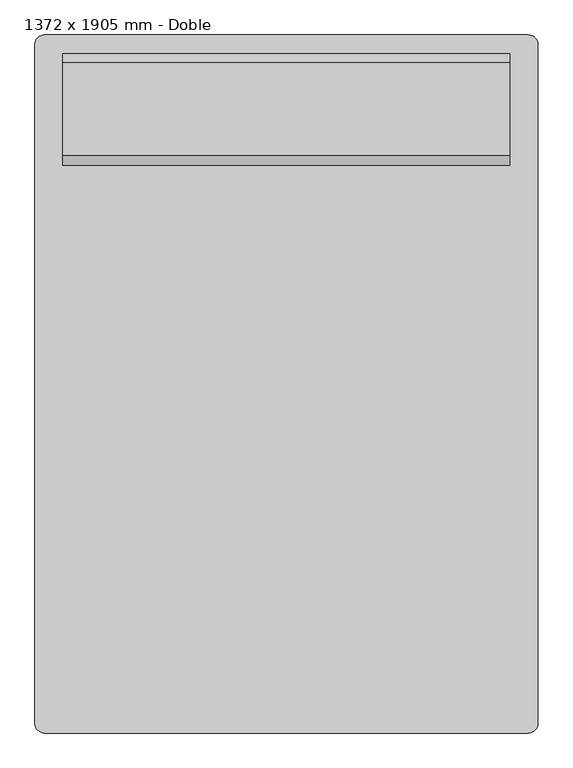
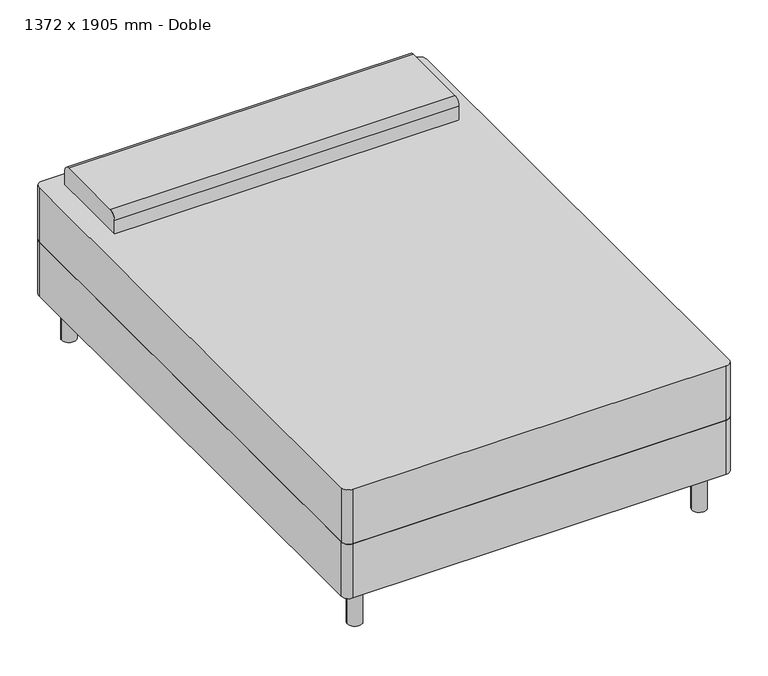
"""IFC4 building model written with IfcOpenShell, lengths in millimetres: furniture geometry, Cama-Estándar : 1372 x 1905 mm - Doble."""

from ifc_helpers import new_model, si_unit, point, frame, frame_2d, origin, origin_with_axes, place, context, project, spatial, polyline, circle_curve, trimmed, segment, composite_curve, outline, extrude, source, transform, mapped, element, save


def furniture_1372_x_1905_mm_doble_2dcc4a2e(model_context):
    return source(origin(), model_context, "Body", "SweptSolid", [
        extrude(outline(composite_curve([segment(polyline([(-414.5114754, -972.695082), (-414.5114754, 881.504918)]), True, "CONTINUOUS"), segment(trimmed(circle_curve(frame_2d((-389.1114754, 881.504918)), 25.4), [point((-414.5114754, 881.504918))], [point((-389.1114754, 906.904918))], False, "CARTESIAN"), True, "CONTINUOUS"), segment(polyline([(-389.1114754, 906.904918), (932.0885246, 906.904918)]), True, "CONTINUOUS"), segment(trimmed(circle_curve(frame_2d((932.0885246, 881.504918)), 25.4), [point((932.0885246, 906.904918))], [point((957.4885246, 881.504918))], False, "CARTESIAN"), True, "CONTINUOUS"), segment(polyline([(957.4885246, 881.504918), (957.4885246, -972.695082)]), True, "CONTINUOUS"), segment(trimmed(circle_curve(frame_2d((932.0885246, -972.695082)), 25.4), [point((957.4885246, -972.695082))], [point((932.0885246, -998.095082))], False, "CARTESIAN"), True, "CONTINUOUS"), segment(polyline([(932.0885246, -998.095082), (-389.1114754, -998.095082)]), True, "CONTINUOUS"), segment(trimmed(circle_curve(frame_2d((-389.1114754, -972.695082)), 25.4), [point((-389.1114754, -998.095082))], [point((-414.5114754, -972.695082))], False, "CARTESIAN"), True, "CONTINUOUS")], self_intersect=False)), frame((0.0, 0.0, 152.4), z_axis=(0.0, 0.0, 1.0), x_axis=(1.0, 0.0, 0.0)), (0.0, 0.0, 1.0), 203.2),
        extrude(outline(composite_curve([segment(polyline([(551.304918, 558.8), (551.304918, 609.6)]), True, "CONTINUOUS"), segment(trimmed(circle_curve(frame_2d((576.704918, 609.6)), 25.4), [point((551.304918, 609.6))], [point((576.704918, 635.0))], False, "CARTESIAN"), True, "CONTINUOUS"), segment(polyline([(576.704918, 635.0), (830.704918, 635.0)]), True, "CONTINUOUS"), segment(trimmed(circle_curve(frame_2d((830.704918, 609.6)), 25.4), [point((830.704918, 635.0))], [point((856.104918, 609.6))], False, "CARTESIAN"), True, "CONTINUOUS"), segment(polyline([(856.104918, 609.6), (856.104918, 558.8), (551.304918, 558.8)]), True, "CONTINUOUS")], self_intersect=False)), frame((-338.3114754, 0.0, 0.0), z_axis=(1.0, 0.0, 0.0), x_axis=(0.0, 1.0, 0.0)), (0.0, 0.0, 1.0), 1219.6),
        extrude(outline(composite_curve([segment(trimmed(circle_curve(frame_2d((-338.3114754, 830.704918)), 25.4), [point((-363.7114754, 830.704918))], [point((-312.9114754, 830.704918))], False, "CARTESIAN"), True, "CONTINUOUS"), segment(trimmed(circle_curve(frame_2d((-338.3114754, 830.704918)), 25.4), [point((-312.9114754, 830.704918))], [point((-363.7114754, 830.704918))], False, "CARTESIAN"), True, "CONTINUOUS")], self_intersect=False)), origin_with_axes(), (0.0, 0.0, 1.0), 152.4),
        extrude(outline(composite_curve([segment(trimmed(circle_curve(frame_2d((881.2885246, 830.704918)), 25.4), [point((855.8885246, 830.704918))], [point((906.6885246, 830.704918))], False, "CARTESIAN"), True, "CONTINUOUS"), segment(trimmed(circle_curve(frame_2d((881.2885246, 830.704918)), 25.4), [point((906.6885246, 830.704918))], [point((855.8885246, 830.704918))], False, "CARTESIAN"), True, "CONTINUOUS")], self_intersect=False)), origin_with_axes(), (0.0, 0.0, 1.0), 152.4),
        extrude(outline(composite_curve([segment(trimmed(circle_curve(frame_2d((881.2885246, -921.895082)), 25.4), [point((855.8885246, -921.895082))], [point((906.6885246, -921.895082))], False, "CARTESIAN"), True, "CONTINUOUS"), segment(trimmed(circle_curve(frame_2d((881.2885246, -921.895082)), 25.4), [point((906.6885246, -921.895082))], [point((855.8885246, -921.895082))], False, "CARTESIAN"), True, "CONTINUOUS")], self_intersect=False)), origin_with_axes(), (0.0, 0.0, 1.0), 152.4),
        extrude(outline(composite_curve([segment(trimmed(circle_curve(frame_2d((-338.3114754, -921.895082)), 25.4), [point((-363.7114754, -921.895082))], [point((-312.9114754, -921.895082))], False, "CARTESIAN"), True, "CONTINUOUS"), segment(trimmed(circle_curve(frame_2d((-338.3114754, -921.895082)), 25.4), [point((-312.9114754, -921.895082))], [point((-363.7114754, -921.895082))], False, "CARTESIAN"), True, "CONTINUOUS")], self_intersect=False)), origin_with_axes(), (0.0, 0.0, 1.0), 152.4),
        extrude(outline(composite_curve([segment(polyline([(-389.1114754, 906.904918), (932.0885246, 906.904918)]), True, "CONTINUOUS"), segment(trimmed(circle_curve(frame_2d((932.0885246, 881.504918)), 25.4), [point((932.0885246, 906.904918))], [point((957.4885246, 881.504918))], False, "CARTESIAN"), True, "CONTINUOUS"), segment(polyline([(957.4885246, 881.504918), (957.4885246, -972.695082)]), True, "CONTINUOUS"), segment(trimmed(circle_curve(frame_2d((932.0885246, -972.695082)), 25.4), [point((957.4885246, -972.695082))], [point((932.0885246, -998.095082))], False, "CARTESIAN"), True, "CONTINUOUS"), segment(polyline([(932.0885246, -998.095082), (-389.1114754, -998.095082)]), True, "CONTINUOUS"), segment(trimmed(circle_curve(frame_2d((-389.1114754, -972.695082)), 25.4), [point((-389.1114754, -998.095082))], [point((-414.5114754, -972.695082))], False, "CARTESIAN"), True, "CONTINUOUS"), segment(polyline([(-414.5114754, -972.695082), (-414.5114754, 881.504918)]), True, "CONTINUOUS"), segment(trimmed(circle_curve(frame_2d((-389.1114754, 881.504918)), 25.4), [point((-414.5114754, 881.504918))], [point((-389.1114754, 906.904918))], False, "CARTESIAN"), True, "CONTINUOUS")], self_intersect=False)), frame((0.0, 0.0, 355.6), z_axis=(0.0, 0.0, 1.0), x_axis=(1.0, 0.0, 0.0)), (0.0, 0.0, 1.0), 203.2),
    ])


if __name__ == "__main__":
    model = new_model("IFC4")
    model_context = context("Model", 3, world=origin())
    ifc_project = project(units=[si_unit("LENGTHUNIT", "METRE", prefix="MILLI")], contexts=[model_context])
    site = spatial("IfcSite", under=ifc_project)
    building = spatial("IfcBuilding", under=site)
    placement = place(None, origin())
    furniture_1372_x_1905_mm_doble_shape = furniture_1372_x_1905_mm_doble_2dcc4a2e(model_context)
    element("IfcFurniture", 1, ObjectType="Cama-Estándar : 1372 x 1905 mm - Doble", at=placement, inside=building, context=model_context, shape_type="MappedRepresentation", body=[
        mapped(furniture_1372_x_1905_mm_doble_shape, transform((0.0, 0.0, 0.0), x_axis=(1.0, 0.0, 0.0), y_axis=(0.0, 1.0, 0.0), z_axis=(0.0, 0.0, 1.0))),
    ])
    save(model, "model.ifc")

# Revit data of these elements
# Project information
#   Subproyecto = "Información de proyecto"
#   Fecha de emisión de proyecto = "Fecha de emisión"
#   Estado de proyecto = "Estado de proyecto"
#   Nombre de cliente = "Propietario"
#   Dirección de proyecto = "Introduzca dirección aquí"
#   Nombre de proyecto = "Nombre de proyecto"
#   Número de proyecto = "0001"
# Type "Cama-Estándar : 1372 x 1905 mm - Doble"
#   Longitud = 1.905 m
#   Anchura = 1.372 m
#   Máscara [instance default] = yes
#   Material de soporte = Metal - Cromo
#   Material de colchón = Textil - Blanco
#   Default Elevation = 0
# Element 1 (IfcFurniture, "Cama-Estándar : 1372 x 1905 mm - Doble")
#   Materials on its faces: "Metal - Cromo", "Textil - Blanco"
# Materials
#   "Metal - Cromo": class "Metal", colour RGB 17 17 17, transparency 0
#   "Textil - Blanco": class "Tela", colour RGB 247 247 239, transparency 0
